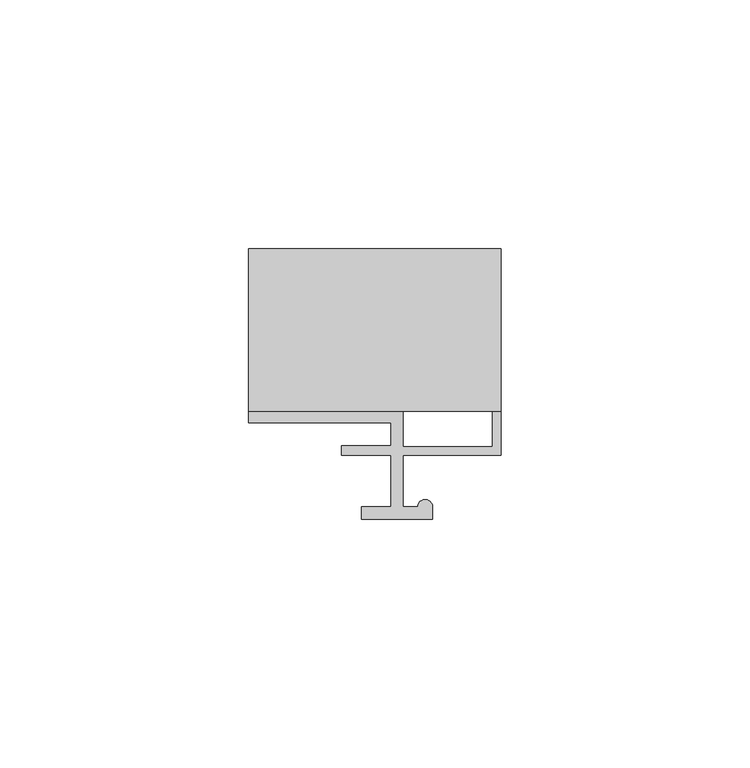
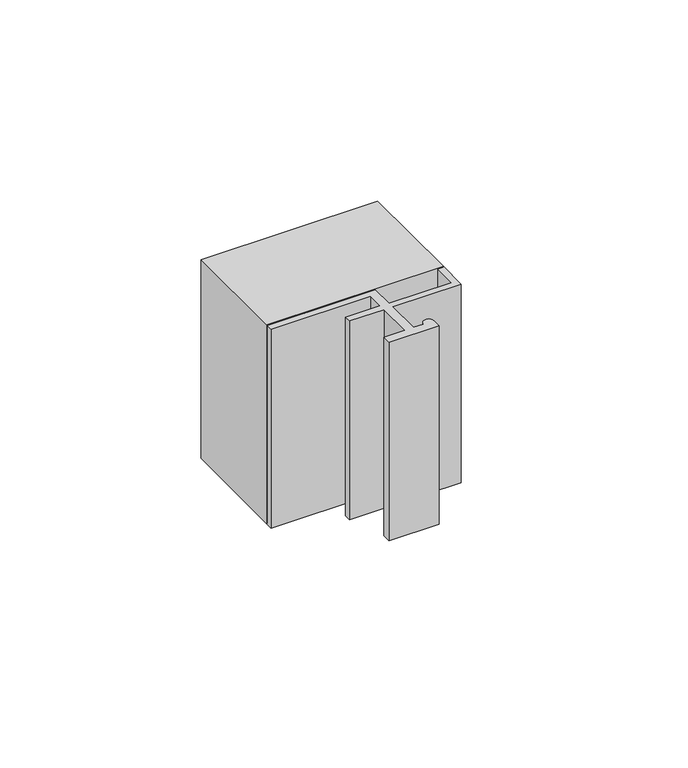
"""IFC4 building model written with IfcOpenShell, lengths in millimetres: proxy geometry, Generic Models 9:Generic Models 5:348123:Generic Models 5:348123 : Generic Models 9:Generic Models 5:348123:2 : Generic Models 9:Generic Models 5:348123:Generic Models 5:348123 : Generic Models 9:Generic Models 5:348123:301771."""

from ifc_helpers import new_model, si_unit, point, frame, frame_2d, origin, place, context, project, spatial, polyline, circle_curve, trimmed, segment, composite_curve, outline, extrude, source, transform, mapped, element, save


def generic_models_676897e9(model_context):
    return source(origin(), model_context, "Body", "SweptSolid", [
        extrude(outline(polyline([(592204.7959377, -579000.6913841), (592255.5959377, -579000.6913841), (592255.5959377, -579033.3483921), (592204.7959377, -579033.3483921), (592204.7959377, -579000.6913841)])), frame((0.0, 0.0, 2462.2125), z_axis=(0.0, 0.0, 1.0), x_axis=(1.0, 0.0, 0.0)), (0.0, 0.0, 1.0), 60.325),
        extrude(outline(composite_curve([segment(polyline([(592235.8677824, -579042.226062), (592235.8677824, -579052.5833435), (592238.8270057, -579052.5833435)]), True, "CONTINUOUS"), segment(trimmed(circle_curve(frame_2d((592240.3066173, -579052.5833435)), 1.4796117), [point((592238.8270057, -579052.5833435))], [point((592241.786229, -579052.5833435))], False, "CARTESIAN"), True, "CONTINUOUS"), segment(polyline([(592241.786229, -579052.5833435), (592241.786229, -579055.0493629), (592227.4833163, -579055.0493629), (592227.4833163, -579052.5833435), (592233.4017629, -579052.5833435), (592233.4017629, -579042.226062), (592223.5376853, -579042.226062), (592223.5376853, -579040.2532464), (592233.4017629, -579040.2532464), (592233.4017629, -579035.6171299), (592204.7959377, -579035.6171299), (592204.7959377, -579033.3483921), (592235.8677824, -579033.3483921), (592235.8677824, -579040.450528), (592253.8204037, -579040.450528), (592253.8204037, -579033.3483921), (592255.5959377, -579033.3483921), (592255.5959377, -579042.226062), (592235.8677824, -579042.226062)]), True, "CONTINUOUS")], self_intersect=False)), frame((0.0, 0.0, 2462.2125), z_axis=(0.0, 0.0, 1.0), x_axis=(1.0, 0.0, 0.0)), (0.0, 0.0, 1.0), 60.325),
    ])


if __name__ == "__main__":
    model = new_model("IFC4")
    model_context = context("Model", 3, world=origin())
    ifc_project = project(units=[si_unit("LENGTHUNIT", "METRE", prefix="MILLI")], contexts=[model_context])
    site = spatial("IfcSite", under=ifc_project)
    building = spatial("IfcBuilding", under=site)
    placement = place(None, origin())
    generic_models_shape = generic_models_676897e9(model_context)
    element("IfcBuildingElementProxy", 1, Name="Generic Models 9:Generic Models 5:348123:Generic Models 5:348123 : Generic Models 9:Generic Models 5:348123:2 : Generic Models 9:Generic Models 5:348123:Generic Models 5:348123 : Generic Models 9:Generic Models 5:348123:301771", ObjectType="Generic Models 9:Generic Models 5:348123:Generic Models 5:348123 : Generic Models 9:Generic Models 5:348123:2 : Generic Models 9:Generic Models 5:348123:Generic Models 5:348123 : Generic Models 9:Generic Models 5:348123:301771", at=placement, inside=building, context=model_context, shape_type="MappedRepresentation", body=[
        mapped(generic_models_shape, transform((0.0, 0.0, 0.0), x_axis=(1.0, 0.0, 0.0), y_axis=(0.0, 1.0, 0.0), z_axis=(0.0, 0.0, 1.0))),
    ])
    save(model, "model.ifc")

# Revit data of these elements
# Type "Generic Models 9:Generic Models 5:348123:Generic Models 5:348123 : Generic Models 9:Generic Models 5:348123:2 : Generic Models 9:Generic Models 5:348123:Generic Models 5:348123 : Generic Models 9:Generic Models 5:348123:301771"
#   NameOverride = "Generic Models 9:Generic Models 5:348123:Generic Models 5:348123 : Generic Models 9:Generic Models 5:348123:301771"
#   ObjectTypeOverride = "Generic Models 5:348123 : Generic Models 9:Generic Models 5:348123"
#   Reference = "Generic Models 5"
#   Tag = "301771"
# Element 1 (IfcBuildingElementProxy, "Generic Models 9:Generic Models 5:348123:Generic Models 5:348123 : Generic Models 9:Generic Models 5:348123:2 : Generic Models 9:Generic Models 5:348123:Generic Models 5:348123 : Generic Models 9:Generic Models 5:348123:301771")
#   Materials on its faces: "GA. STEEL CLIP AT EVERY SEAM IN POLYCARBONATE (WITH STEEL PLATE EXTENSION, IF NECS.)"
# Materials
#   "GA. STEEL CLIP AT EVERY SEAM IN POLYCARBONATE (WITH STEEL PLATE EXTENSION, IF NECS.)": class "Unassigned", colour RGB 120 120 120, transparency 0, Cost = 0
